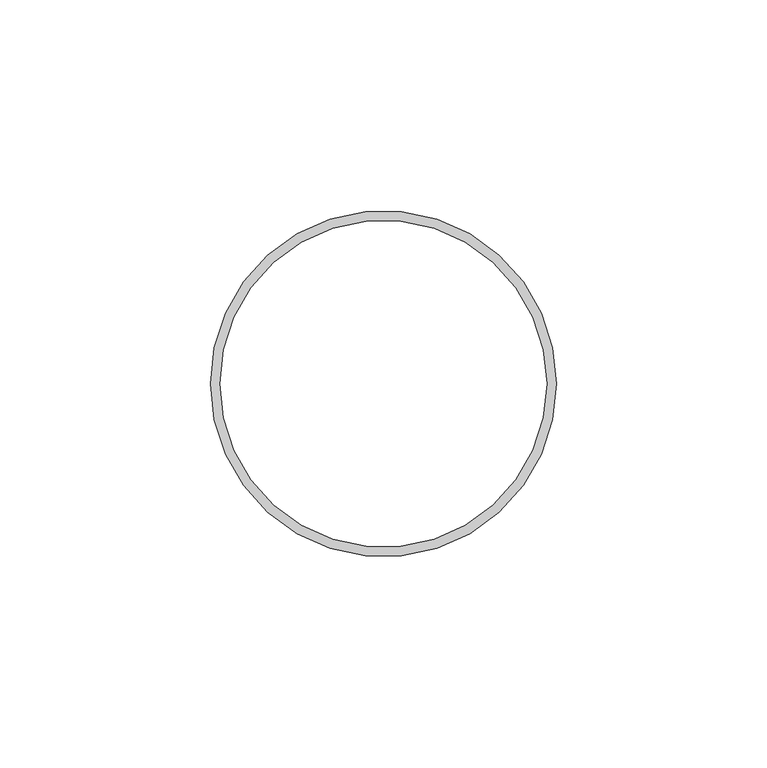
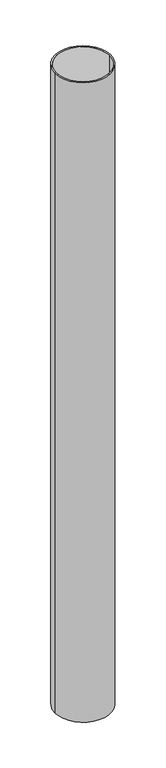
"""IFC4 building model written with IfcOpenShell, lengths in millimetres: proxy geometry, TN_ПВС 125-82_Водосточная труба : TN_ПВС 125-82_Водосточная труба."""

from ifc_helpers import new_model, si_unit, point, origin, origin_with_axes, origin_2d, place, context, project, spatial, circle_curve, trimmed, segment, composite_curve, outline, extrude, source, transform, mapped, element, save


def generic_models_eecc9471(model_context):
    return source(origin(), model_context, "Body", "SweptSolid", [
        extrude(outline(composite_curve([segment(trimmed(circle_curve(origin_2d(), 41.1), [point((-41.1, 0.0))], [point((41.1, 0.0))], False, "CARTESIAN"), True, "CONTINUOUS"), segment(trimmed(circle_curve(origin_2d(), 41.1), [point((41.1, 0.0))], [point((-41.1, 0.0))], False, "CARTESIAN"), True, "CONTINUOUS")], self_intersect=False), holes=[composite_curve([segment(trimmed(circle_curve(origin_2d(), 38.8), [point((-38.8, 0.0))], [point((38.8, 0.0))], True, "CARTESIAN"), True, "CONTINUOUS"), segment(trimmed(circle_curve(origin_2d(), 38.8), [point((38.8, 0.0))], [point((-38.8, 0.0))], True, "CARTESIAN"), True, "CONTINUOUS")], self_intersect=False)]), origin_with_axes(), (0.0, 0.0, 1.0), 1000.0),
    ])


if __name__ == "__main__":
    model = new_model("IFC4")
    model_context = context("Model", 3, world=origin())
    ifc_project = project(units=[si_unit("LENGTHUNIT", "METRE", prefix="MILLI")], contexts=[model_context])
    site = spatial("IfcSite", under=ifc_project)
    building = spatial("IfcBuilding", under=site)
    placement = place(None, origin())
    generic_models_shape = generic_models_eecc9471(model_context)
    element("IfcBuildingElementProxy", 1, Name="TN_ПВС 125-82_Водосточная труба : TN_ПВС 125-82_Водосточная труба", ObjectType="TN_ПВС 125-82_Водосточная труба : TN_ПВС 125-82_Водосточная труба", at=placement, inside=building, context=model_context, shape_type="MappedRepresentation", body=[
        mapped(generic_models_shape, transform((0.0, 0.0, 0.0), x_axis=(1.0, 0.0, 0.0), y_axis=(0.0, 1.0, 0.0), z_axis=(0.0, 0.0, 1.0))),
    ])
    save(model, "model.ifc")

# Revit data of these elements
# Type "TN_ПВС 125-82_Водосточная труба : TN_ПВС 125-82_Водосточная труба"
#   Description = "Организует вертикальный сток дождевой воды"
#   Manufacturer = "ТехноНИКОЛЬ"
#   Model = "Комплектующие к водосточным системам"
#   URL = "https://tn-vodostok.ru/catalog/pvh/"
#   ADSK_Обозначение = "ТехноНИКОЛЬ"
#   ADSK_Наименование краткое = "Труба"
#   ADSK_Наименование = "Водосточная труба"
#   ADSK_Масса_Текст = ""
#   ADSK_Марка = ""
#   ADSK_Код изделия = ""
#   ADSK_Завод-изготовитель = "ТехноНИКОЛЬ"
#   ADSK_Единица измерения = "п.м."
#   ADSK_Группирование = "Комплектующие к водосточным системам"
#   ADSK_URL страницы изделия = "https://tn-vodostok.ru/catalog/pvh/"
#   ADSK_URL документации изделия = "https://tn-vodostok.ru/upload/iblock/c42/c427963cb77eb5c3c51f0cfb870e9e52.pdf"
#   ADSK_Размер_Диаметр = 82.2 mm
#   ADSK_Размер_Высота [instance default] = 500 mm
#   ADSK_Количество [instance default] = 0.5
#   ADSK_Материал [instance default] = TN_Пластик_Коричневый_RAL8019
#   Default Elevation = 0
# Element 1 (IfcBuildingElementProxy, "TN_ПВС 125-82_Водосточная труба : TN_ПВС 125-82_Водосточная труба")
#   ADSK_Размер_Высота = 1000 mm
#   ADSK_Количество = 1
#   Materials on its faces: "TN_Пластик_Коричневый_RAL8019"
# Materials
#   "TN_Пластик_Коричневый_RAL8019": class "Типовые", colour RGB 61 54 53, transparency 0, Cost = 0
